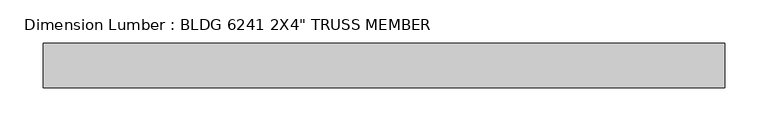
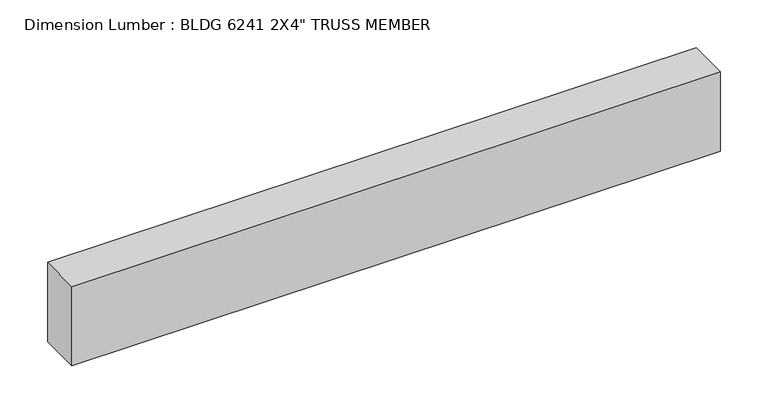
"""IFC4 building model written with IfcOpenShell, lengths in millimetres: beam geometry."""

from ifc_helpers import new_model, si_unit, frame, origin, place, context, project, spatial, polyline, outline, extrude, source, transform, mapped, element, save


def beam_ce158ae4(model_context):
    return source(origin(), model_context, "Body", "SweptSolid", [
        extrude(outline(polyline([(392.1124994, 25.4), (392.1124994, -25.4), (-392.1125, -25.4), (-392.1125, 25.4), (392.1124994, 25.4)])), frame((0.0, 0.0, -50.8), z_axis=(0.0, 0.0, 1.0), x_axis=(1.0, 0.0, 0.0)), (0.0, 0.0, 1.0), 101.6),
    ])


if __name__ == "__main__":
    model = new_model("IFC4")
    model_context = context("Model", 3, world=origin())
    ifc_project = project(units=[si_unit("LENGTHUNIT", "METRE", prefix="MILLI")], contexts=[model_context])
    site = spatial("IfcSite", under=ifc_project)
    building = spatial("IfcBuilding", under=site)
    placement = place(None, origin())
    beam_shape = beam_ce158ae4(model_context)
    element("IfcBeam", 1, ObjectType="Dimension Lumber : BLDG 6241 2X4\" TRUSS MEMBER", at=placement, inside=building, context=model_context, shape_type="MappedRepresentation", body=[
        mapped(beam_shape, transform((0.0, 0.0, 0.0), x_axis=(1.0, 0.0, 0.0), y_axis=(0.0, 1.0, 0.0), z_axis=(0.0, 0.0, 1.0))),
    ])
    save(model, "model.ifc")

# Revit data of these elements
# Type "Dimension Lumber : BLDG 6241 2X4\" TRUSS MEMBER"
#   Assembly Code = "B10"
#   A = 0.273472 SF
#   Length [instance default] = 5' - 0"
#   b = 0' - 2"
#   d = 0' - 4"
#   Structural Material [instance default] = Softwood, Lumber
# Element 1 (IfcBeam, "Dimension Lumber : BLDG 6241 2X4\" TRUSS MEMBER")
#   Materials on its faces: "Softwood, Lumber"
# Materials
#   "Softwood, Lumber": class "Wood", colour RGB 223 192 134, transparency 0, Description = "Pinus Echinata", Cost = 0
